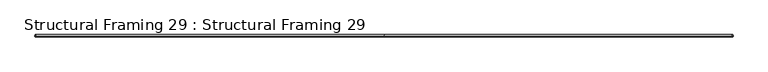
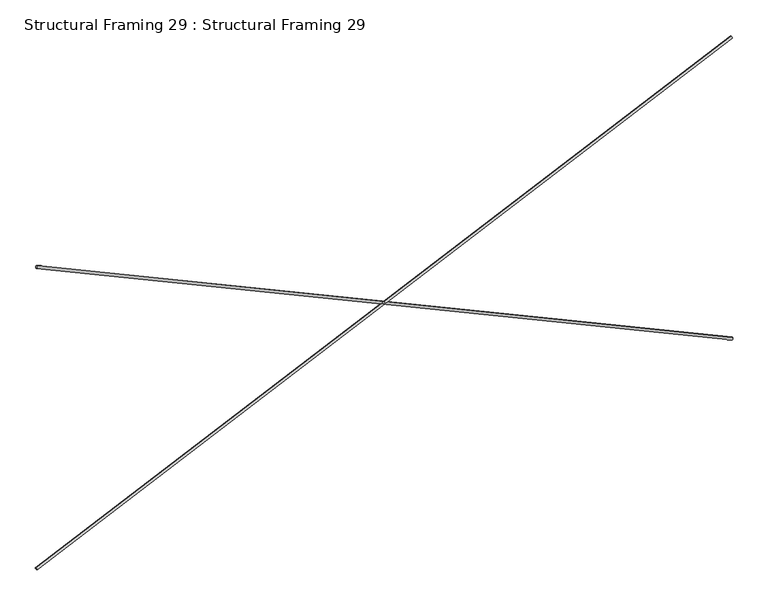
"""IFC4 building model written with IfcOpenShell, lengths in millimetres: beam geometry, Structural Framing 29 : Structural Framing 29."""

from ifc_helpers import new_model, si_unit, point, frame, origin, origin_2d, place, context, project, spatial, circle_curve, trimmed, segment, composite_curve, outline, extrude, source, transform, mapped, element, save


def structural_framing_29_structural_framing_29_66df7c48(model_context):
    return source(origin(), model_context, "Body", "SweptSolid", [
        extrude(outline(composite_curve([segment(trimmed(circle_curve(origin_2d(), 9.525), [point((0.0, 9.525))], [point((0.0, -9.525))], False, "CARTESIAN"), True, "CONTINUOUS"), segment(trimmed(circle_curve(origin_2d(), 9.525), [point((0.0, -9.525))], [point((0.0, 9.525))], False, "CARTESIAN"), True, "CONTINUOUS")], self_intersect=False)), frame((17917.0574817, 2611.1115366, 18.7589856), z_axis=(-0.9087990366403788, 0.0, 0.4172341201310358), x_axis=(0.0, 1.0, 0.0)), (0.0, 0.0, 1.0), 5816.6),
        extrude(outline(composite_curve([segment(trimmed(circle_curve(origin_2d(), 9.525), [point((0.0, -9.525))], [point((0.0, 9.525))], False, "CARTESIAN"), True, "CONTINUOUS"), segment(trimmed(circle_curve(origin_2d(), 9.525), [point((0.0, 9.525))], [point((0.0, -9.525))], False, "CARTESIAN"), True, "CONTINUOUS")], self_intersect=False)), frame((12628.0165287, 2611.1115366, 18.7589856), z_axis=(0.9087990366403788, 0.0, 0.4172341201310358), x_axis=(0.0, 1.0, 0.0)), (0.0, 0.0, 1.0), 5816.6),
    ])


if __name__ == "__main__":
    model = new_model("IFC4")
    model_context = context("Model", 3, world=origin())
    ifc_project = project(units=[si_unit("LENGTHUNIT", "METRE", prefix="MILLI")], contexts=[model_context])
    site = spatial("IfcSite", under=ifc_project)
    building = spatial("IfcBuilding", under=site)
    placement = place(None, origin())
    structural_framing_29_structural_framing_29_shape = structural_framing_29_structural_framing_29_66df7c48(model_context)
    element("IfcBeam", 1, ObjectType="Structural Framing 29 : Structural Framing 29", at=placement, inside=building, context=model_context, shape_type="MappedRepresentation", body=[
        mapped(structural_framing_29_structural_framing_29_shape, transform((0.0, 0.0, 0.0), x_axis=(1.0, 0.0, 0.0), y_axis=(0.0, 1.0, 0.0), z_axis=(0.0, 0.0, 1.0))),
    ])
    save(model, "model.ifc")

# Revit data of these elements
# Element 1 (IfcBeam, "Structural Framing 29 : Structural Framing 29")
#   Materials on its faces: "X-BRACING: 3/4\" DIA. THREADED STEEL ROD (RAW) W/ TURNBUCKLE (NUTS AT STEEL ANGLE)"
# Materials
#   "X-BRACING: 3/4\" DIA. THREADED STEEL ROD (RAW) W/ TURNBUCKLE (NUTS AT STEEL ANGLE)": class "Generic", colour RGB 212 212 212, transparency 0, Cost = 0
